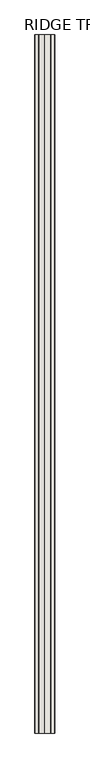
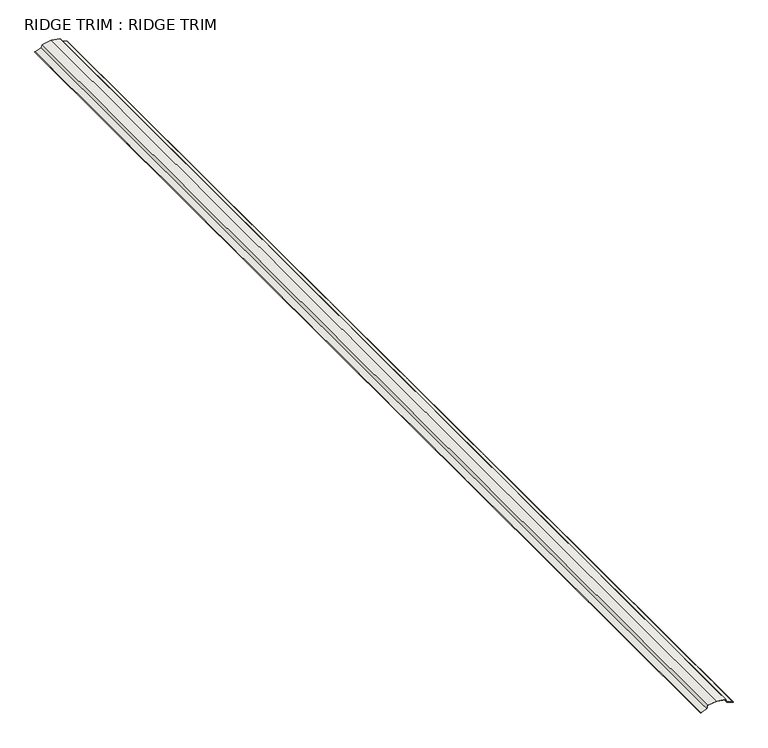
"""IFC4 building model written with IfcOpenShell, lengths in millimetres: wall geometry, RIDGE TRIM : RIDGE TRIM."""

from ifc_helpers import new_model, si_unit, point, frame, frame_2d, origin, place, context, project, spatial, polyline, circle_curve, trimmed, segment, composite_curve, outline, extrude, source, transform, mapped, element, save


def ridge_trim_ridge_trim_c9808429(model_context):
    return source(origin(), model_context, "Body", "SweptSolid", [
        extrude(outline(composite_curve([segment(polyline([(5914.1050494, 21357.2744185), (5884.2286097, 21346.0816767), (5864.635531, 21286.3527082)]), True, "CONTINUOUS"), segment(trimmed(circle_curve(frame_2d((5862.3729069, 21287.0949238)), 2.38125), [point((5864.635531, 21286.3527082))], [point((5860.1102829, 21287.8371394))], False, "CARTESIAN"), True, "CONTINUOUS"), segment(polyline([(5860.1102829, 21287.8371394), (5863.5391209, 21298.2898591), (5865.047537, 21297.7950487), (5861.6186989, 21287.342329)]), True, "CONTINUOUS"), segment(trimmed(circle_curve(frame_2d((5862.3729069, 21287.0949238)), 0.79375), [point((5861.6186989, 21287.342329))], [point((5863.1271149, 21286.8475186))], True, "CARTESIAN"), True, "CONTINUOUS"), segment(polyline([(5863.1271149, 21286.8475186), (5882.9578042, 21347.3008363), (5912.6898278, 21358.4394749), (5927.1107218, 21444.9648383), (5912.6898278, 21531.4902018), (5882.9578042, 21542.6288404), (5862.7593268, 21602.9602697)]), True, "CONTINUOUS"), segment(trimmed(circle_curve(frame_2d((5862.0066394, 21602.7082761)), 0.79375), [point((5862.7593268, 21602.9602697))], [point((5861.253952, 21602.4562824))], True, "CARTESIAN"), True, "CONTINUOUS"), segment(polyline([(5861.253952, 21602.4562824), (5864.7463828, 21592.0246378), (5863.2410081, 21591.5206505), (5859.7485773, 21601.952295)]), True, "CONTINUOUS"), segment(trimmed(circle_curve(frame_2d((5862.0066394, 21602.7082761)), 2.38125), [point((5859.7485773, 21601.952295))], [point((5864.2647015, 21603.4642571))], False, "CARTESIAN"), True, "CONTINUOUS"), segment(polyline([(5864.2647015, 21603.4642571), (5884.2230473, 21543.8500838), (5914.1050494, 21532.6552582), (5928.7201193, 21444.9648383), (5914.1050494, 21357.2744185)]), True, "CONTINUOUS")], self_intersect=False)), frame((0.0, -4202.4384634, 0.0), z_axis=(0.0, 1.0, 0.0), x_axis=(0.0, 0.0, 1.0)), (0.0, 0.0, 1.0), 11315.7),
    ])


if __name__ == "__main__":
    model = new_model("IFC4")
    model_context = context("Model", 3, world=origin())
    ifc_project = project(units=[si_unit("LENGTHUNIT", "METRE", prefix="MILLI")], contexts=[model_context])
    site = spatial("IfcSite", under=ifc_project)
    building = spatial("IfcBuilding", under=site)
    placement = place(None, origin())
    ridge_trim_ridge_trim_shape = ridge_trim_ridge_trim_c9808429(model_context)
    element("IfcWall", 1, ObjectType="RIDGE TRIM : RIDGE TRIM", at=placement, inside=building, context=model_context, shape_type="MappedRepresentation", body=[
        mapped(ridge_trim_ridge_trim_shape, transform((0.0, 0.0, 0.0), x_axis=(1.0, 0.0, 0.0), y_axis=(0.0, 1.0, 0.0), z_axis=(0.0, 0.0, 1.0))),
    ])
    save(model, "model.ifc")

# Revit data of these elements
# Element 1 (IfcWall, "RIDGE TRIM : RIDGE TRIM")
#   Materials on its faces: "RIDGE TRIM"
# Materials
#   "RIDGE TRIM": class "Generic", colour RGB 195 195 195, transparency 0, Cost = 0
